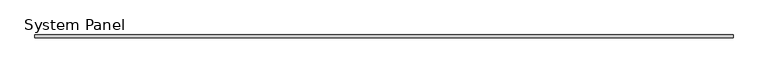
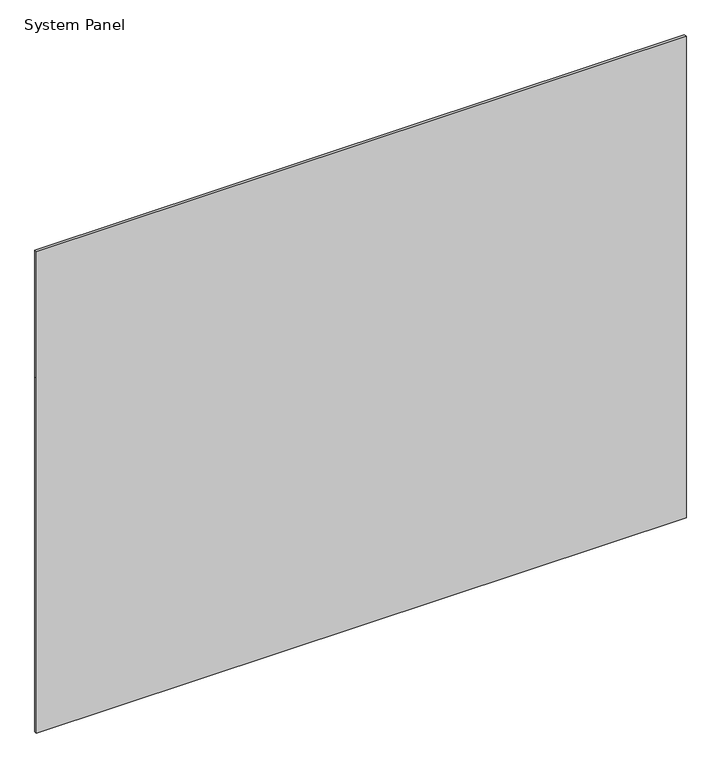
"""IFC4 building model written with IfcOpenShell, lengths in millimetres: plate geometry, System Panel : 로이복층유리_16."""

from ifc_helpers import new_model, si_unit, frame, origin, place, context, project, spatial, polyline, outline, extrude, source, transform, mapped, element, save


def system_panel_bb32a1b4(model_context):
    return source(origin(), model_context, "Body", "SweptSolid", [
        extrude(outline(polyline([(0.0, -1887.5), (0.0, 1887.5), (2177.5, 1887.5), (2955.0, 1887.5), (2955.0, -1887.5), (2177.5, -1887.5), (0.0, -1887.5)])), frame((0.0, -8.0, 0.0), z_axis=(0.0, 1.0, 0.0), x_axis=(0.0, 0.0, 1.0)), (0.0, 0.0, 1.0), 16.0),
    ])


if __name__ == "__main__":
    model = new_model("IFC4")
    model_context = context("Model", 3, world=origin())
    ifc_project = project(units=[si_unit("LENGTHUNIT", "METRE", prefix="MILLI")], contexts=[model_context])
    site = spatial("IfcSite", under=ifc_project)
    building = spatial("IfcBuilding", under=site)
    placement = place(None, origin())
    system_panel_shape = system_panel_bb32a1b4(model_context)
    element("IfcPlate", 1, ObjectType="System Panel : 로이복층유리_16", at=placement, inside=building, context=model_context, shape_type="MappedRepresentation", body=[
        mapped(system_panel_shape, transform((0.0, 0.0, 0.0), x_axis=(1.0, 0.0, 0.0), y_axis=(0.0, 1.0, 0.0), z_axis=(0.0, 0.0, 1.0))),
    ])
    save(model, "model.ifc")

# Revit data of these elements
# Element 1 (IfcPlate, "System Panel : 로이복층유리_16")
#   Materials on its faces: "00_Glass_Glass"
# Materials
#   "00_Glass_Glass": class "Glass", colour RGB 218 227 224, transparency 0.85, Description = "Glass", Cost = 0, Image = none
